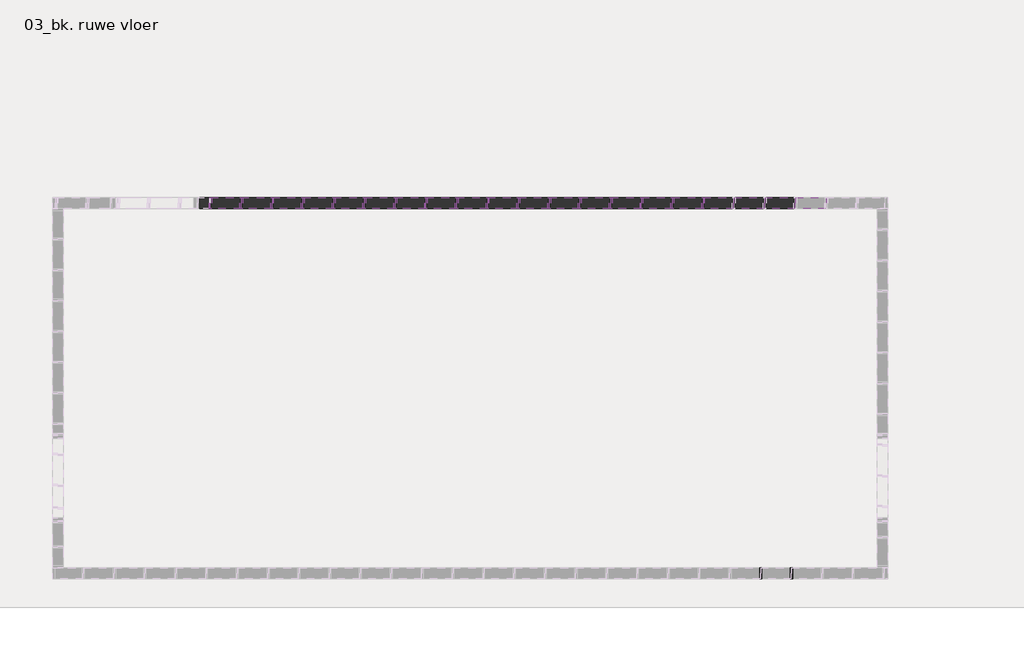
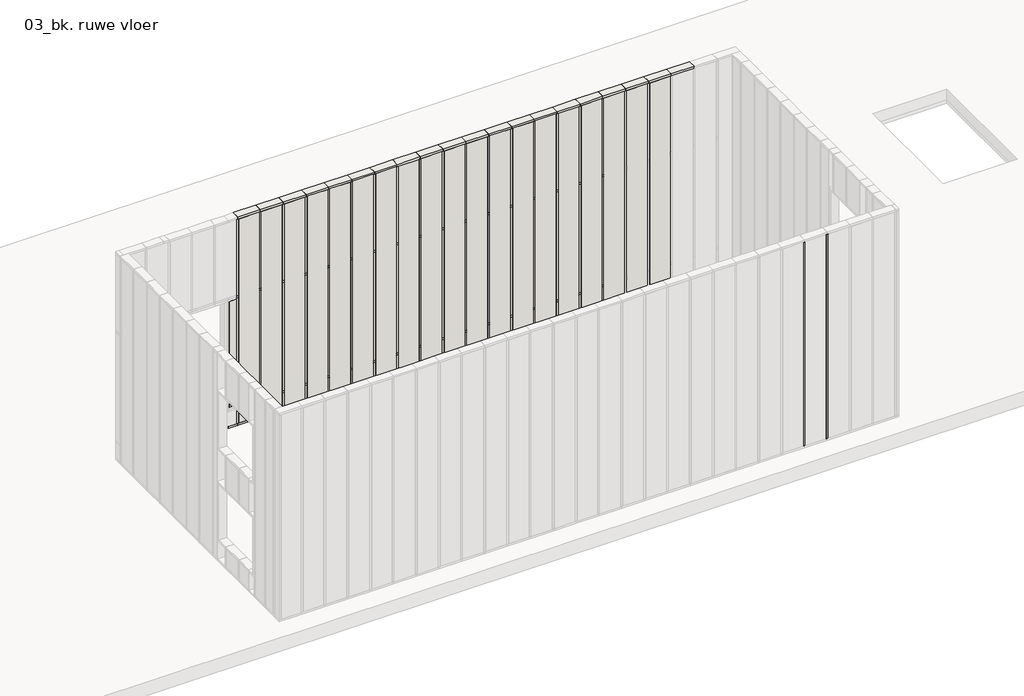
# One storey, part 3 of 9: 144 walls.
# Revit data of these elements (continued)
# Type "Rectangular Mullion : NLRS_21_CWM_hsb-regel 38x142_gen_rsf"
#   Type IfcGUID = "07M7mRoiH1CR8m_RSKIwpF"
#   Assembly Code = "21.10"
#   IfcExportAs = "IfcWall"
#   built-in parameter 1007322 = 0.465879 (stored number, unit not read)
#   built-in parameter 1007321 = 0.062336 (stored number, unit not read)
#   built-in parameter 1007320 = 0.062336 (stored number, unit not read)
# Type "System Panel : NLRS_21_CWP_hsb-vulling minerale wol 142 _gen_rsf"
#   Type IfcGUID = "07M7mRoiH1CR8m_RSKIwpC"
#   Assembly Code = "21.23"
#   IfcExportAs = "IfcWall"
# Element 1 (IfcWall, "Rectangular Mullion : NLRS_21_CWM_hsb-regel 38x142_gen_rsf")
#   IfcGUID = "07M7mRoiH1CR8m_RSKIwQK"
#   IsExternal = yes
#   LoadBearing = yes
#   Phase Created = NLRS_nieuw
#   Materials on its faces: "NLRS_i2_hout naaldhout vuren_gen_rsf"
# Element 2 (IfcWall, "Rectangular Mullion : NLRS_21_CWM_hsb-regel 38x142_gen_rsf")
#   IfcGUID = "07M7mRoiH1CR8m_RSKIwQR"
#   IsExternal = yes
#   LoadBearing = yes
#   Phase Created = NLRS_nieuw
#   Materials on its faces: "NLRS_i2_hout naaldhout vuren_gen_rsf"
# Element 3 (IfcWall, "Rectangular Mullion : NLRS_21_CWM_hsb-regel 38x142_gen_rsf")
#   IfcGUID = "07M7mRoiH1CR8m_RSKIwQQ"
#   IsExternal = yes
#   LoadBearing = yes
#   Phase Created = NLRS_nieuw
#   Materials on its faces: "NLRS_i2_hout naaldhout vuren_gen_rsf"
# Element 4 (IfcWall, "Rectangular Mullion : NLRS_21_CWM_hsb-regel 38x142_gen_rsf")
#   IfcGUID = "07M7mRoiH1CR8m_RSKIwQP"
#   IsExternal = yes
#   LoadBearing = yes
#   Phase Created = NLRS_nieuw
#   Materials on its faces: "NLRS_i2_hout naaldhout vuren_gen_rsf"
# Element 5 (IfcWall, "Rectangular Mullion : NLRS_21_CWM_hsb-regel 38x142_gen_rsf")
#   IfcGUID = "07M7mRoiH1CR8m_RSKIwQO"
#   IsExternal = yes
#   LoadBearing = yes
#   Phase Created = NLRS_nieuw
#   Materials on its faces: "NLRS_i2_hout naaldhout vuren_gen_rsf"
# Element 6 (IfcWall, "Rectangular Mullion : NLRS_21_CWM_hsb-regel 38x142_gen_rsf")
#   IfcGUID = "07M7mRoiH1CR8m_RSKIwQV"
#   IsExternal = yes
#   LoadBearing = yes
#   Phase Created = NLRS_nieuw
#   Materials on its faces: "NLRS_i2_hout naaldhout vuren_gen_rsf"
# Element 7 (IfcWall, "Rectangular Mullion : NLRS_21_CWM_hsb-regel 38x142_gen_rsf")
#   IfcGUID = "07M7mRoiH1CR8m_RSKIwQU"
#   IsExternal = yes
#   LoadBearing = yes
#   Phase Created = NLRS_nieuw
#   Materials on its faces: "NLRS_i2_hout naaldhout vuren_gen_rsf"
# Element 8 (IfcWall, "Rectangular Mullion : NLRS_21_CWM_hsb-regel 38x142_gen_rsf")
#   IfcGUID = "07M7mRoiH1CR8m_RSKIwQT"
#   IsExternal = yes
#   LoadBearing = yes
#   Phase Created = NLRS_nieuw
#   Materials on its faces: "NLRS_i2_hout naaldhout vuren_gen_rsf"
# Element 9 (IfcWall, "Rectangular Mullion : NLRS_21_CWM_hsb-regel 38x142_gen_rsf")
#   IfcGUID = "07M7mRoiH1CR8m_RSKIwQS"
#   IsExternal = yes
#   LoadBearing = yes
#   Phase Created = NLRS_nieuw
#   Materials on its faces: "NLRS_i2_hout naaldhout vuren_gen_rsf"
# Element 10 (IfcWall, "Rectangular Mullion : NLRS_21_CWM_hsb-regel 38x142_gen_rsf")
#   IfcGUID = "07M7mRoiH1CR8m_RSKIwPZ"
#   IsExternal = yes
#   LoadBearing = yes
#   Phase Created = NLRS_nieuw
#   Materials on its faces: "NLRS_i2_hout naaldhout vuren_gen_rsf"
# Element 11 (IfcWall, "Rectangular Mullion : NLRS_21_CWM_hsb-regel 38x142_gen_rsf")
#   IfcGUID = "07M7mRoiH1CR8m_RSKIwPY"
#   IsExternal = yes
#   LoadBearing = yes
#   Phase Created = NLRS_nieuw
#   Materials on its faces: "NLRS_i2_hout naaldhout vuren_gen_rsf"
# Element 12 (IfcWall, "Rectangular Mullion : NLRS_21_CWM_hsb-regel 38x142_gen_rsf")
#   IfcGUID = "07M7mRoiH1CR8m_RSKIwPX"
#   IsExternal = yes
#   LoadBearing = yes
#   Phase Created = NLRS_nieuw
#   Materials on its faces: "NLRS_i2_hout naaldhout vuren_gen_rsf"
# Element 13 (IfcWall, "Rectangular Mullion : NLRS_21_CWM_hsb-regel 38x142_gen_rsf")
#   IfcGUID = "07M7mRoiH1CR8m_RSKIwPW"
#   IsExternal = yes
#   LoadBearing = yes
#   Phase Created = NLRS_nieuw
#   Materials on its faces: "NLRS_i2_hout naaldhout vuren_gen_rsf"
# Element 14 (IfcWall, "Rectangular Mullion : NLRS_21_CWM_hsb-regel 38x142_gen_rsf")
#   IfcGUID = "07M7mRoiH1CR8m_RSKIwPd"
#   IsExternal = yes
#   LoadBearing = yes
#   Phase Created = NLRS_nieuw
#   Materials on its faces: "NLRS_i2_hout naaldhout vuren_gen_rsf"
# Element 15 (IfcWall, "Rectangular Mullion : NLRS_21_CWM_hsb-regel 38x142_gen_rsf")
#   IfcGUID = "07M7mRoiH1CR8m_RSKIwPc"
#   IsExternal = yes
#   LoadBearing = yes
#   Phase Created = NLRS_nieuw
#   Materials on its faces: "NLRS_i2_hout naaldhout vuren_gen_rsf"
# Element 16 (IfcWall, "Rectangular Mullion : NLRS_21_CWM_hsb-regel 38x142_gen_rsf")
#   IfcGUID = "07M7mRoiH1CR8m_RSKIwPb"
#   IsExternal = yes
#   LoadBearing = yes
#   Phase Created = NLRS_nieuw
#   Materials on its faces: "NLRS_i2_hout naaldhout vuren_gen_rsf"
# Element 17 (IfcWall, "Rectangular Mullion : NLRS_21_CWM_hsb-regel 38x142_gen_rsf")
#   IfcGUID = "07M7mRoiH1CR8m_RSKIwPa"
#   IsExternal = yes
#   LoadBearing = yes
#   Phase Created = NLRS_nieuw
#   Materials on its faces: "NLRS_i2_hout naaldhout vuren_gen_rsf"
# Element 18 (IfcWall, "Rectangular Mullion : NLRS_21_CWM_hsb-regel 38x142_gen_rsf")
#   IfcGUID = "07M7mRoiH1CR8m_RSKIwUD"
#   IsExternal = yes
#   LoadBearing = yes
#   Phase Created = NLRS_nieuw
#   Materials on its faces: "NLRS_i2_hout naaldhout vuren_gen_rsf"
# Element 19 (IfcWall, "Rectangular Mullion : NLRS_21_CWM_hsb-regel 38x142_gen_rsf")
#   IfcGUID = "07M7mRoiH1CR8m_RSKIwUC"
#   IsExternal = yes
#   LoadBearing = yes
#   Phase Created = NLRS_nieuw
#   Materials on its faces: "NLRS_i2_hout naaldhout vuren_gen_rsf"
# Element 20 (IfcWall, "Rectangular Mullion : NLRS_21_CWM_hsb-regel 38x142_gen_rsf")
#   IfcGUID = "07M7mRoiH1CR8m_RSKIwIM"
#   IsExternal = yes
#   LoadBearing = yes
#   Phase Created = NLRS_nieuw
#   Materials on its faces: "NLRS_i2_hout naaldhout vuren_gen_rsf"
# Element 21 (IfcWall, "Rectangular Mullion : NLRS_21_CWM_hsb-regel 38x142_gen_rsf")
#   IfcGUID = "07M7mRoiH1CR8m_RSKIwPj"
#   IsExternal = yes
#   LoadBearing = yes
#   Phase Created = NLRS_nieuw
#   Materials on its faces: "NLRS_i2_hout naaldhout vuren_gen_rsf"
# Element 22 (IfcWall, "Rectangular Mullion : NLRS_21_CWM_hsb-regel 38x142_gen_rsf")
#   IfcGUID = "07M7mRoiH1CR8m_RSKIwPi"
#   IsExternal = yes
#   LoadBearing = yes
#   Phase Created = NLRS_nieuw
#   Materials on its faces: "NLRS_i2_hout naaldhout vuren_gen_rsf"
# Element 23 (IfcWall, "Rectangular Mullion : NLRS_21_CWM_hsb-regel 38x142_gen_rsf")
#   IfcGUID = "07M7mRoiH1CR8m_RSKIwPp"
#   IsExternal = yes
#   LoadBearing = yes
#   Phase Created = NLRS_nieuw
#   Materials on its faces: "NLRS_i2_hout naaldhout vuren_gen_rsf"
# Element 24 (IfcWall, "Rectangular Mullion : NLRS_21_CWM_hsb-regel 38x142_gen_rsf")
#   IfcGUID = "07M7mRoiH1CR8m_RSKIwPo"
#   IsExternal = yes
#   LoadBearing = yes
#   Phase Created = NLRS_nieuw
#   Materials on its faces: "NLRS_i2_hout naaldhout vuren_gen_rsf"
# Element 25 (IfcWall, "Rectangular Mullion : NLRS_21_CWM_hsb-regel 38x142_gen_rsf")
#   IfcGUID = "07M7mRoiH1CR8m_RSKIwPn"
#   IsExternal = yes
#   LoadBearing = yes
#   Phase Created = NLRS_nieuw
#   Materials on its faces: "NLRS_i2_hout naaldhout vuren_gen_rsf"
# Element 26 (IfcWall, "Rectangular Mullion : NLRS_21_CWM_hsb-regel 38x142_gen_rsf")
#   IfcGUID = "07M7mRoiH1CR8m_RSKIwPm"
#   IsExternal = yes
#   LoadBearing = yes
#   Phase Created = NLRS_nieuw
#   Materials on its faces: "NLRS_i2_hout naaldhout vuren_gen_rsf"
# Element 27 (IfcWall, "Rectangular Mullion : NLRS_21_CWM_hsb-regel 38x142_gen_rsf")
#   IfcGUID = "07M7mRoiH1CR8m_RSKIwPt"
#   IsExternal = yes
#   LoadBearing = yes
#   Phase Created = NLRS_nieuw
#   Materials on its faces: "NLRS_i2_hout naaldhout vuren_gen_rsf"
# Element 28 (IfcWall, "Rectangular Mullion : NLRS_21_CWM_hsb-regel 38x142_gen_rsf")
#   IfcGUID = "07M7mRoiH1CR8m_RSKIwPs"
#   IsExternal = yes
#   LoadBearing = yes
#   Phase Created = NLRS_nieuw
#   Materials on its faces: "NLRS_i2_hout naaldhout vuren_gen_rsf"
# Element 29 (IfcWall, "Rectangular Mullion : NLRS_21_CWM_hsb-regel 38x142_gen_rsf")
#   IfcGUID = "07M7mRoiH1CR8m_RSKIwPr"
#   IsExternal = yes
#   LoadBearing = yes
#   Phase Created = NLRS_nieuw
#   Materials on its faces: "NLRS_i2_hout naaldhout vuren_gen_rsf"
# Element 30 (IfcWall, "Rectangular Mullion : NLRS_21_CWM_hsb-regel 38x142_gen_rsf")
#   IfcGUID = "07M7mRoiH1CR8m_RSKIwPq"
#   IsExternal = yes
#   LoadBearing = yes
#   Phase Created = NLRS_nieuw
#   Materials on its faces: "NLRS_i2_hout naaldhout vuren_gen_rsf"
# Element 31 (IfcWall, "Rectangular Mullion : NLRS_21_CWM_hsb-regel 38x142_gen_rsf")
#   IfcGUID = "07M7mRoiH1CR8m_RSKIwPx"
#   IsExternal = yes
#   LoadBearing = yes
#   Phase Created = NLRS_nieuw
#   Materials on its faces: "NLRS_i2_hout naaldhout vuren_gen_rsf"
# Element 32 (IfcWall, "Rectangular Mullion : NLRS_21_CWM_hsb-regel 38x142_gen_rsf")
#   IfcGUID = "07M7mRoiH1CR8m_RSKIwPw"
#   IsExternal = yes
#   LoadBearing = yes
#   Phase Created = NLRS_nieuw
#   Materials on its faces: "NLRS_i2_hout naaldhout vuren_gen_rsf"
# Element 33 (IfcWall, "Rectangular Mullion : NLRS_21_CWM_hsb-regel 38x142_gen_rsf")
#   IfcGUID = "07M7mRoiH1CR8m_RSKIwPv"
#   IsExternal = yes
#   LoadBearing = yes
#   Phase Created = NLRS_nieuw
#   Materials on its faces: "NLRS_i2_hout naaldhout vuren_gen_rsf"
# Element 34 (IfcWall, "Rectangular Mullion : NLRS_21_CWM_hsb-regel 38x142_gen_rsf")
#   IfcGUID = "07M7mRoiH1CR8m_RSKIwPu"
#   IsExternal = yes
#   LoadBearing = yes
#   Phase Created = NLRS_nieuw
#   Materials on its faces: "NLRS_i2_hout naaldhout vuren_gen_rsf"
# Element 35 (IfcWall, "Rectangular Mullion : NLRS_21_CWM_hsb-regel 38x142_gen_rsf")
#   IfcGUID = "07M7mRoiH1CR8m_RSKIwUJ"
#   IsExternal = yes
#   LoadBearing = yes
#   Phase Created = NLRS_nieuw
#   Materials on its faces: "NLRS_i2_hout naaldhout vuren_gen_rsf"
# Element 36 (IfcWall, "Rectangular Mullion : NLRS_21_CWM_hsb-regel 38x142_gen_rsf")
#   IfcGUID = "3JRv6RmLn4$9gi2tFo70EI"
#   IsExternal = yes
#   LoadBearing = yes
#   Phase Created = NLRS_nieuw
#   Materials on its faces: "NLRS_i2_hout naaldhout vuren_gen_rsf"
# Element 37 (IfcWall, "Rectangular Mullion : NLRS_21_CWM_hsb-regel 38x142_gen_rsf")
#   IfcGUID = "07M7mRoiH1CR8m_RSKIwIY"
#   IsExternal = yes
#   LoadBearing = yes
#   Phase Created = NLRS_nieuw
#   Materials on its faces: "NLRS_i2_hout naaldhout vuren_gen_rsf"
# Element 38 (IfcWall, "Rectangular Mullion : NLRS_21_CWM_hsb-regel 38x142_gen_rsf")
#   IfcGUID = "07M7mRoiH1CR8m_RSKIwIX"
#   IsExternal = yes
#   LoadBearing = yes
#   Phase Created = NLRS_nieuw
#   Materials on its faces: "NLRS_i2_hout naaldhout vuren_gen_rsf"
# Element 39 (IfcWall, "Rectangular Mullion : NLRS_21_CWM_hsb-regel 38x142_gen_rsf")
#   IfcGUID = "07M7mRoiH1CR8m_RSKIwP0"
#   IsExternal = yes
#   LoadBearing = yes
#   Phase Created = NLRS_nieuw
#   Materials on its faces: "NLRS_i2_hout naaldhout vuren_gen_rsf"
# Element 40 (IfcWall, "Rectangular Mullion : NLRS_21_CWM_hsb-regel 38x142_gen_rsf")
#   IfcGUID = "07M7mRoiH1CR8m_RSKIwP7"
#   IsExternal = yes
#   LoadBearing = yes
#   Phase Created = NLRS_nieuw
#   Materials on its faces: "NLRS_i2_hout naaldhout vuren_gen_rsf"
# Element 41 (IfcWall, "Rectangular Mullion : NLRS_21_CWM_hsb-regel 38x142_gen_rsf")
#   IfcGUID = "07M7mRoiH1CR8m_RSKIwP6"
#   IsExternal = yes
#   LoadBearing = yes
#   Phase Created = NLRS_nieuw
#   Materials on its faces: "NLRS_i2_hout naaldhout vuren_gen_rsf"
# Element 42 (IfcWall, "Rectangular Mullion : NLRS_21_CWM_hsb-regel 38x142_gen_rsf")
#   IfcGUID = "07M7mRoiH1CR8m_RSKIwP5"
#   IsExternal = yes
#   LoadBearing = yes
#   Phase Created = NLRS_nieuw
#   Materials on its faces: "NLRS_i2_hout naaldhout vuren_gen_rsf"
# Element 43 (IfcWall, "Rectangular Mullion : NLRS_21_CWM_hsb-regel 38x142_gen_rsf")
#   IfcGUID = "07M7mRoiH1CR8m_RSKIwP4"
#   IsExternal = yes
#   LoadBearing = yes
#   Phase Created = NLRS_nieuw
#   Materials on its faces: "NLRS_i2_hout naaldhout vuren_gen_rsf"
# Element 44 (IfcWall, "Rectangular Mullion : NLRS_21_CWM_hsb-regel 38x142_gen_rsf")
#   IfcGUID = "07M7mRoiH1CR8m_RSKIwPB"
#   IsExternal = yes
#   LoadBearing = yes
#   Phase Created = NLRS_nieuw
#   Materials on its faces: "NLRS_i2_hout naaldhout vuren_gen_rsf"
# Element 45 (IfcWall, "Rectangular Mullion : NLRS_21_CWM_hsb-regel 38x142_gen_rsf")
#   IfcGUID = "07M7mRoiH1CR8m_RSKIwPA"
#   IsExternal = yes
#   LoadBearing = yes
#   Phase Created = NLRS_nieuw
#   Materials on its faces: "NLRS_i2_hout naaldhout vuren_gen_rsf"
# Element 46 (IfcWall, "Rectangular Mullion : NLRS_21_CWM_hsb-regel 38x142_gen_rsf")
#   IfcGUID = "07M7mRoiH1CR8m_RSKIwP9"
#   IsExternal = yes
#   LoadBearing = yes
#   Phase Created = NLRS_nieuw
#   Materials on its faces: "NLRS_i2_hout naaldhout vuren_gen_rsf"
# Element 47 (IfcWall, "Rectangular Mullion : NLRS_21_CWM_hsb-regel 38x142_gen_rsf")
#   IfcGUID = "07M7mRoiH1CR8m_RSKIwP8"
#   IsExternal = yes
#   LoadBearing = yes
#   Phase Created = NLRS_nieuw
#   Materials on its faces: "NLRS_i2_hout naaldhout vuren_gen_rsf"
# Element 48 (IfcWall, "Rectangular Mullion : NLRS_21_CWM_hsb-regel 38x142_gen_rsf")
#   IfcGUID = "07M7mRoiH1CR8m_RSKIwPF"
#   IsExternal = yes
#   LoadBearing = yes
#   Phase Created = NLRS_nieuw
#   Materials on its faces: "NLRS_i2_hout naaldhout vuren_gen_rsf"
# Element 49 (IfcWall, "Rectangular Mullion : NLRS_21_CWM_hsb-regel 38x142_gen_rsf")
#   IfcGUID = "07M7mRoiH1CR8m_RSKIwPE"
#   IsExternal = yes
#   LoadBearing = yes
#   Phase Created = NLRS_nieuw
#   Materials on its faces: "NLRS_i2_hout naaldhout vuren_gen_rsf"
# Element 50 (IfcWall, "Rectangular Mullion : NLRS_21_CWM_hsb-regel 38x142_gen_rsf")
#   IfcGUID = "07M7mRoiH1CR8m_RSKIwPD"
#   IsExternal = yes
#   LoadBearing = yes
#   Phase Created = NLRS_nieuw
#   Materials on its faces: "NLRS_i2_hout naaldhout vuren_gen_rsf"
# Element 51 (IfcWall, "Rectangular Mullion : NLRS_21_CWM_hsb-regel 38x142_gen_rsf")
#   IfcGUID = "07M7mRoiH1CR8m_RSKIwPC"
#   IsExternal = yes
#   LoadBearing = yes
#   Phase Created = NLRS_nieuw
#   Materials on its faces: "NLRS_i2_hout naaldhout vuren_gen_rsf"
# Element 52 (IfcWall, "Rectangular Mullion : NLRS_21_CWM_hsb-regel 38x142_gen_rsf")
#   IfcGUID = "07M7mRoiH1CR8m_RSKIwPJ"
#   IsExternal = yes
#   LoadBearing = yes
#   Phase Created = NLRS_nieuw
#   Materials on its faces: "NLRS_i2_hout naaldhout vuren_gen_rsf"
# Element 53 (IfcWall, "Rectangular Mullion : NLRS_21_CWM_hsb-regel 38x142_gen_rsf")
#   IfcGUID = "07M7mRoiH1CR8m_RSKIwUI"
#   IsExternal = yes
#   LoadBearing = yes
#   Phase Created = NLRS_nieuw
#   Materials on its faces: "NLRS_i2_hout naaldhout vuren_gen_rsf"
# Element 54 (IfcWall, "Rectangular Mullion : NLRS_21_CWM_hsb-regel 38x142_gen_rsf")
#   IfcGUID = "07M7mRoiH1CR8m_RSKIwUH"
#   IsExternal = yes
#   LoadBearing = yes
#   Phase Created = NLRS_nieuw
#   Materials on its faces: "NLRS_i2_hout naaldhout vuren_gen_rsf"
# Element 55 (IfcWall, "Rectangular Mullion : NLRS_21_CWM_hsb-regel 38x142_gen_rsf")
#   IfcGUID = "07M7mRoiH1CR8m_RSKIwHY"
#   IsExternal = yes
#   LoadBearing = yes
#   Phase Created = NLRS_nieuw
#   Materials on its faces: "NLRS_i2_hout naaldhout vuren_gen_rsf"
# Element 56 (IfcWall, "Rectangular Mullion : NLRS_21_CWM_hsb-regel 38x142_gen_rsf")
#   IfcGUID = "3JRv6RmLn4$9gi2tFo70EJ"
#   IsExternal = yes
#   LoadBearing = yes
#   Phase Created = NLRS_nieuw
#   Materials on its faces: "NLRS_i2_hout naaldhout vuren_gen_rsf"
# Element 57 (IfcWall, "Rectangular Mullion : NLRS_21_CWM_hsb-regel 38x142_gen_rsf")
#   IfcGUID = "3JRv6RmLn4$9gi2tFo70WL"
#   IsExternal = yes
#   LoadBearing = yes
#   Phase Created = NLRS_nieuw
#   Materials on its faces: "NLRS_i2_hout naaldhout vuren_gen_rsf"
# Element 58 (IfcWall, "Rectangular Mullion : NLRS_21_CWM_hsb-regel 38x142_gen_rsf")
#   IfcGUID = "3JRv6RmLn4$9gi2tFo70WM"
#   IsExternal = yes
#   LoadBearing = yes
#   Phase Created = NLRS_nieuw
#   Materials on its faces: "NLRS_i2_hout naaldhout vuren_gen_rsf"
# Element 59 (IfcWall, "Rectangular Mullion : NLRS_21_CWM_hsb-regel 38x142_gen_rsf")
#   IfcGUID = "3JRv6RmLn4$9gi2tFo70WN"
#   IsExternal = yes
#   LoadBearing = yes
#   Phase Created = NLRS_nieuw
#   Materials on its faces: "NLRS_i2_hout naaldhout vuren_gen_rsf"
# Element 60 (IfcWall, "Rectangular Mullion : NLRS_21_CWM_hsb-regel 38x142_gen_rsf")
#   IfcGUID = "3JRv6RmLn4$9gi2tFo70WG"
#   IsExternal = yes
#   LoadBearing = yes
#   Phase Created = NLRS_nieuw
#   Materials on its faces: "NLRS_i2_hout naaldhout vuren_gen_rsf"
# Element 61 (IfcWall, "Rectangular Mullion : NLRS_21_CWM_hsb-regel 38x142_gen_rsf")
#   IfcGUID = "3JRv6RmLn4$9gi2tFo70WH"
#   IsExternal = yes
#   LoadBearing = yes
#   Phase Created = NLRS_nieuw
#   Materials on its faces: "NLRS_i2_hout naaldhout vuren_gen_rsf"
# Element 62 (IfcWall, "Rectangular Mullion : NLRS_21_CWM_hsb-regel 38x142_gen_rsf")
#   IfcGUID = "3JRv6RmLn4$9gi2tFo70WI"
#   IsExternal = yes
#   LoadBearing = yes
#   Phase Created = NLRS_nieuw
#   Materials on its faces: "NLRS_i2_hout naaldhout vuren_gen_rsf"
# Element 63 (IfcWall, "Rectangular Mullion : NLRS_21_CWM_hsb-regel 38x142_gen_rsf")
#   IfcGUID = "3JRv6RmLn4$9gi2tFo70WJ"
#   IsExternal = yes
#   LoadBearing = yes
#   Phase Created = NLRS_nieuw
#   Materials on its faces: "NLRS_i2_hout naaldhout vuren_gen_rsf"
# Element 64 (IfcWall, "Rectangular Mullion : NLRS_21_CWM_hsb-regel 38x142_gen_rsf")
#   IfcGUID = "3JRv6RmLn4$9gi2tFo70WS"
#   IsExternal = yes
#   LoadBearing = yes
#   Phase Created = NLRS_nieuw
#   Materials on its faces: "NLRS_i2_hout naaldhout vuren_gen_rsf"
# Element 65 (IfcWall, "Rectangular Mullion : NLRS_21_CWM_hsb-regel 38x142_gen_rsf")
#   IfcGUID = "3JRv6RmLn4$9gi2tFo70WT"
#   IsExternal = yes
#   LoadBearing = yes
#   Phase Created = NLRS_nieuw
#   Materials on its faces: "NLRS_i2_hout naaldhout vuren_gen_rsf"
# Element 66 (IfcWall, "Rectangular Mullion : NLRS_21_CWM_hsb-regel 38x142_gen_rsf")
#   IfcGUID = "3JRv6RmLn4$9gi2tFo70WU"
#   IsExternal = yes
#   LoadBearing = yes
#   Phase Created = NLRS_nieuw
#   Materials on its faces: "NLRS_i2_hout naaldhout vuren_gen_rsf"
# Element 67 (IfcWall, "Rectangular Mullion : NLRS_21_CWM_hsb-regel 38x142_gen_rsf")
#   IfcGUID = "3JRv6RmLn4$9gi2tFo70WV"
#   IsExternal = yes
#   LoadBearing = yes
#   Phase Created = NLRS_nieuw
#   Materials on its faces: "NLRS_i2_hout naaldhout vuren_gen_rsf"
# Element 68 (IfcWall, "Rectangular Mullion : NLRS_21_CWM_hsb-regel 38x142_gen_rsf")
#   IfcGUID = "3JRv6RmLn4$9gi2tFo70WO"
#   IsExternal = yes
#   LoadBearing = yes
#   Phase Created = NLRS_nieuw
#   Materials on its faces: "NLRS_i2_hout naaldhout vuren_gen_rsf"
# Element 69 (IfcWall, "Rectangular Mullion : NLRS_21_CWM_hsb-regel 38x142_gen_rsf")
#   IfcGUID = "3JRv6RmLn4$9gi2tFo70WP"
#   IsExternal = yes
#   LoadBearing = yes
#   Phase Created = NLRS_nieuw
#   Materials on its faces: "NLRS_i2_hout naaldhout vuren_gen_rsf"
# Element 70 (IfcWall, "Rectangular Mullion : NLRS_21_CWM_hsb-regel 38x142_gen_rsf")
#   IfcGUID = "3JRv6RmLn4$9gi2tFo70WQ"
#   IsExternal = yes
#   LoadBearing = yes
#   Phase Created = NLRS_nieuw
#   Materials on its faces: "NLRS_i2_hout naaldhout vuren_gen_rsf"
# Element 71 (IfcWall, "Rectangular Mullion : NLRS_21_CWM_hsb-regel 38x142_gen_rsf")
#   IfcGUID = "3JRv6RmLn4$9gi2tFo70WR"
#   IsExternal = yes
#   LoadBearing = yes
#   Phase Created = NLRS_nieuw
#   Materials on its faces: "NLRS_i2_hout naaldhout vuren_gen_rsf"
# Element 72 (IfcWall, "Rectangular Mullion : NLRS_21_CWM_hsb-regel 38x142_gen_rsf")
#   IfcGUID = "3JRv6RmLn4$9gi2tFo70Xa"
#   IsExternal = yes
#   LoadBearing = yes
#   Phase Created = NLRS_nieuw
#   Materials on its faces: "NLRS_i2_hout naaldhout vuren_gen_rsf"
# Element 73 (IfcWall, "Rectangular Mullion : NLRS_21_CWM_hsb-regel 38x142_gen_rsf")
#   IfcGUID = "3JRv6RmLn4$9gi2tFo70Xb"
#   IsExternal = yes
#   LoadBearing = yes
#   Phase Created = NLRS_nieuw
#   Materials on its faces: "NLRS_i2_hout naaldhout vuren_gen_rsf"
# Element 74 (IfcWall, "Rectangular Mullion : NLRS_21_CWM_hsb-regel 38x142_gen_rsf")
#   IfcGUID = "3JRv6RmLn4$9gi2tFo70wj"
#   IsExternal = yes
#   LoadBearing = yes
#   Phase Created = NLRS_nieuw
#   Materials on its faces: "NLRS_i2_hout naaldhout vuren_gen_rsf"
# Element 75 (IfcWall, "Rectangular Mullion : NLRS_21_CWM_hsb-regel 38x142_gen_rsf")
#   IfcGUID = "3JRv6RmLn4$9gi2tFo70wk"
#   IsExternal = yes
#   LoadBearing = yes
#   Phase Created = NLRS_nieuw
#   Materials on its faces: "NLRS_i2_hout naaldhout vuren_gen_rsf"
# Element 76 (IfcWall, "Rectangular Mullion : NLRS_21_CWM_hsb-regel 38x142_gen_rsf")
#   IfcGUID = "3JRv6RmLn4$9gi2tFo70wl"
#   IsExternal = yes
#   LoadBearing = yes
#   Phase Created = NLRS_nieuw
#   Materials on its faces: "NLRS_i2_hout naaldhout vuren_gen_rsf"
# Element 77 (IfcWall, "Rectangular Mullion : NLRS_21_CWM_hsb-regel 38x142_gen_rsf")
#   IfcGUID = "3JRv6RmLn4$9gi2tFo70we"
#   IsExternal = yes
#   LoadBearing = yes
#   Phase Created = NLRS_nieuw
#   Materials on its faces: "NLRS_i2_hout naaldhout vuren_gen_rsf"
# Element 78 (IfcWall, "Rectangular Mullion : NLRS_21_CWM_hsb-regel 38x142_gen_rsf")
#   IfcGUID = "3JRv6RmLn4$9gi2tFo70wf"
#   IsExternal = yes
#   LoadBearing = yes
#   Phase Created = NLRS_nieuw
#   Materials on its faces: "NLRS_i2_hout naaldhout vuren_gen_rsf"
# Element 79 (IfcWall, "Rectangular Mullion : NLRS_21_CWM_hsb-regel 38x142_gen_rsf")
#   IfcGUID = "3JRv6RmLn4$9gi2tFo70wg"
#   IsExternal = yes
#   LoadBearing = yes
#   Phase Created = NLRS_nieuw
#   Materials on its faces: "NLRS_i2_hout naaldhout vuren_gen_rsf"
# Element 80 (IfcWall, "Rectangular Mullion : NLRS_21_CWM_hsb-regel 38x142_gen_rsf")
#   IfcGUID = "3JRv6RmLn4$9gi2tFo70wh"
#   IsExternal = yes
#   LoadBearing = yes
#   Phase Created = NLRS_nieuw
#   Materials on its faces: "NLRS_i2_hout naaldhout vuren_gen_rsf"
# Element 81 (IfcWall, "Rectangular Mullion : NLRS_21_CWM_hsb-regel 38x142_gen_rsf")
#   IfcGUID = "3JRv6RmLn4$9gi2tFo70wq"
#   IsExternal = yes
#   LoadBearing = yes
#   Phase Created = NLRS_nieuw
#   Materials on its faces: "NLRS_i2_hout naaldhout vuren_gen_rsf"
# Element 82 (IfcWall, "Rectangular Mullion : NLRS_21_CWM_hsb-regel 38x142_gen_rsf")
#   IfcGUID = "3JRv6RmLn4$9gi2tFo70wr"
#   IsExternal = yes
#   LoadBearing = yes
#   Phase Created = NLRS_nieuw
#   Materials on its faces: "NLRS_i2_hout naaldhout vuren_gen_rsf"
# Element 83 (IfcWall, "Rectangular Mullion : NLRS_21_CWM_hsb-regel 38x142_gen_rsf")
#   IfcGUID = "3JRv6RmLn4$9gi2tFo70ws"
#   IsExternal = yes
#   LoadBearing = yes
#   Phase Created = NLRS_nieuw
#   Materials on its faces: "NLRS_i2_hout naaldhout vuren_gen_rsf"
# Element 84 (IfcWall, "Rectangular Mullion : NLRS_21_CWM_hsb-regel 38x142_gen_rsf")
#   IfcGUID = "3JRv6RmLn4$9gi2tFo70wt"
#   IsExternal = yes
#   LoadBearing = yes
#   Phase Created = NLRS_nieuw
#   Materials on its faces: "NLRS_i2_hout naaldhout vuren_gen_rsf"
# Element 85 (IfcWall, "Rectangular Mullion : NLRS_21_CWM_hsb-regel 38x142_gen_rsf")
#   IfcGUID = "3JRv6RmLn4$9gi2tFo70wm"
#   IsExternal = yes
#   LoadBearing = yes
#   Phase Created = NLRS_nieuw
#   Materials on its faces: "NLRS_i2_hout naaldhout vuren_gen_rsf"
# Element 86 (IfcWall, "Rectangular Mullion : NLRS_21_CWM_hsb-regel 38x142_gen_rsf")
#   IfcGUID = "3JRv6RmLn4$9gi2tFo70wn"
#   IsExternal = yes
#   LoadBearing = yes
#   Phase Created = NLRS_nieuw
#   Materials on its faces: "NLRS_i2_hout naaldhout vuren_gen_rsf"
# Element 87 (IfcWall, "Rectangular Mullion : NLRS_21_CWM_hsb-regel 38x142_gen_rsf")
#   IfcGUID = "3JRv6RmLn4$9gi2tFo70wo"
#   IsExternal = yes
#   LoadBearing = yes
#   Phase Created = NLRS_nieuw
#   Materials on its faces: "NLRS_i2_hout naaldhout vuren_gen_rsf"
# Element 88 (IfcWall, "Rectangular Mullion : NLRS_21_CWM_hsb-regel 38x142_gen_rsf")
#   IfcGUID = "3JRv6RmLn4$9gi2tFo70wp"
#   IsExternal = yes
#   LoadBearing = yes
#   Phase Created = NLRS_nieuw
#   Materials on its faces: "NLRS_i2_hout naaldhout vuren_gen_rsf"
# Element 89 (IfcWall, "Rectangular Mullion : NLRS_21_CWM_hsb-regel 38x142_gen_rsf")
#   IfcGUID = "3JRv6RmLn4$9gi2tFo70wy"
#   IsExternal = yes
#   LoadBearing = yes
#   Phase Created = NLRS_nieuw
#   Materials on its faces: "NLRS_i2_hout naaldhout vuren_gen_rsf"
# Element 90 (IfcWall, "Rectangular Mullion : NLRS_21_CWM_hsb-regel 38x142_gen_rsf")
#   IfcGUID = "3JRv6RmLn4$9gi2tFo70hi"
#   IsExternal = yes
#   LoadBearing = yes
#   Phase Created = NLRS_nieuw
#   Materials on its faces: "NLRS_i2_hout naaldhout vuren_gen_rsf"
# Element 91 (IfcWall, "Rectangular Mullion : NLRS_21_CWM_hsb-regel 38x142_gen_rsf")
#   IfcGUID = "3JRv6RmLn4$9gi2tFo70hj"
#   IsExternal = yes
#   LoadBearing = yes
#   Phase Created = NLRS_nieuw
#   Materials on its faces: "NLRS_i2_hout naaldhout vuren_gen_rsf"
# Element 92 (IfcWall, "Rectangular Mullion : NLRS_21_CWM_hsb-regel 38x142_gen_rsf")
#   IfcGUID = "3JRv6RmLn4$9gi2tFo70hk"
#   IsExternal = yes
#   LoadBearing = yes
#   Phase Created = NLRS_nieuw
#   Materials on its faces: "NLRS_i2_hout naaldhout vuren_gen_rsf"
# Element 93 (IfcWall, "Rectangular Mullion : NLRS_21_CWM_hsb-regel 38x142_gen_rsf")
#   IfcGUID = "3JRv6RmLn4$9gi2tFo70hl"
#   IsExternal = yes
#   LoadBearing = yes
#   Phase Created = NLRS_nieuw
#   Materials on its faces: "NLRS_i2_hout naaldhout vuren_gen_rsf"
# Element 94 (IfcWall, "Rectangular Mullion : NLRS_21_CWM_hsb-regel 38x142_gen_rsf")
#   IfcGUID = "3JRv6RmLn4$9gi2tFo70he"
#   IsExternal = yes
#   LoadBearing = yes
#   Phase Created = NLRS_nieuw
#   Materials on its faces: "NLRS_i2_hout naaldhout vuren_gen_rsf"
# Element 95 (IfcWall, "Rectangular Mullion : NLRS_21_CWM_hsb-regel 38x142_gen_rsf")
#   IfcGUID = "3JRv6RmLn4$9gi2tFo70hf"
#   IsExternal = yes
#   LoadBearing = yes
#   Phase Created = NLRS_nieuw
#   Materials on its faces: "NLRS_i2_hout naaldhout vuren_gen_rsf"
# Element 96 (IfcWall, "Rectangular Mullion : NLRS_21_CWM_hsb-regel 38x142_gen_rsf")
#   IfcGUID = "3JRv6RmLn4$9gi2tFo70hg"
#   IsExternal = yes
#   LoadBearing = yes
#   Phase Created = NLRS_nieuw
#   Materials on its faces: "NLRS_i2_hout naaldhout vuren_gen_rsf"
# Element 97 (IfcWall, "Rectangular Mullion : NLRS_21_CWM_hsb-regel 38x142_gen_rsf")
#   IfcGUID = "3JRv6RmLn4$9gi2tFo70hh"
#   IsExternal = yes
#   LoadBearing = yes
#   Phase Created = NLRS_nieuw
#   Materials on its faces: "NLRS_i2_hout naaldhout vuren_gen_rsf"
# Element 98 (IfcWall, "Rectangular Mullion : NLRS_21_CWM_hsb-regel 38x142_gen_rsf")
#   IfcGUID = "3JRv6RmLn4$9gi2tFo70hq"
#   IsExternal = yes
#   LoadBearing = yes
#   Phase Created = NLRS_nieuw
#   Materials on its faces: "NLRS_i2_hout naaldhout vuren_gen_rsf"
# Element 99 (IfcWall, "Rectangular Mullion : NLRS_21_CWM_hsb-regel 38x142_gen_rsf")
#   IfcGUID = "3JRv6RmLn4$9gi2tFo70hr"
#   IsExternal = yes
#   LoadBearing = yes
#   Phase Created = NLRS_nieuw
#   Materials on its faces: "NLRS_i2_hout naaldhout vuren_gen_rsf"
# Element 100 (IfcWall, "Rectangular Mullion : NLRS_21_CWM_hsb-regel 38x142_gen_rsf")
#   IfcGUID = "3JRv6RmLn4$9gi2tFo70hs"
#   IsExternal = yes
#   LoadBearing = yes
#   Phase Created = NLRS_nieuw
#   Materials on its faces: "NLRS_i2_hout naaldhout vuren_gen_rsf"
# Element 101 (IfcWall, "Rectangular Mullion : NLRS_21_CWM_hsb-regel 38x142_gen_rsf")
#   IfcGUID = "3JRv6RmLn4$9gi2tFo70ht"
#   IsExternal = yes
#   LoadBearing = yes
#   Phase Created = NLRS_nieuw
#   Materials on its faces: "NLRS_i2_hout naaldhout vuren_gen_rsf"
# Element 102 (IfcWall, "Rectangular Mullion : NLRS_21_CWM_hsb-regel 38x142_gen_rsf")
#   IfcGUID = "3JRv6RmLn4$9gi2tFo70hm"
#   IsExternal = yes
#   LoadBearing = yes
#   Phase Created = NLRS_nieuw
#   Materials on its faces: "NLRS_i2_hout naaldhout vuren_gen_rsf"
# Element 103 (IfcWall, "Rectangular Mullion : NLRS_21_CWM_hsb-regel 38x142_gen_rsf")
#   IfcGUID = "3JRv6RmLn4$9gi2tFo70hn"
#   IsExternal = yes
#   LoadBearing = yes
#   Phase Created = NLRS_nieuw
#   Materials on its faces: "NLRS_i2_hout naaldhout vuren_gen_rsf"
# Element 104 (IfcWall, "Rectangular Mullion : NLRS_21_CWM_hsb-regel 38x142_gen_rsf")
#   IfcGUID = "3JRv6RmLn4$9gi2tFo70ho"
#   IsExternal = yes
#   LoadBearing = yes
#   Phase Created = NLRS_nieuw
#   Materials on its faces: "NLRS_i2_hout naaldhout vuren_gen_rsf"
# Element 105 (IfcWall, "Rectangular Mullion : NLRS_21_CWM_hsb-regel 38x142_gen_rsf")
#   IfcGUID = "3JRv6RmLn4$9gi2tFo70hp"
#   IsExternal = yes
#   LoadBearing = yes
#   Phase Created = NLRS_nieuw
#   Materials on its faces: "NLRS_i2_hout naaldhout vuren_gen_rsf"
# Element 106 (IfcWall, "Rectangular Mullion : NLRS_21_CWM_hsb-regel 38x142_gen_rsf")
#   IfcGUID = "3JRv6RmLn4$9gi2tFo70wz"
#   IsExternal = yes
#   LoadBearing = yes
#   Phase Created = NLRS_nieuw
#   Materials on its faces: "NLRS_i2_hout naaldhout vuren_gen_rsf"
# Element 107 (IfcWall, "Rectangular Mullion : NLRS_21_CWM_hsb-regel 38x142_gen_rsf")
#   IfcGUID = "3JRv6RmLn4$9gi2tFo70hy"
#   IsExternal = yes
#   LoadBearing = yes
#   Phase Created = NLRS_nieuw
#   Materials on its faces: "NLRS_i2_hout naaldhout vuren_gen_rsf"
# Element 108 (IfcWall, "Rectangular Mullion : NLRS_21_CWM_hsb-regel 38x142_gen_rsf")
#   IfcGUID = "3JRv6RmLn4$9gi2tFo70kv"
#   IsExternal = yes
#   LoadBearing = yes
#   Phase Created = NLRS_nieuw
#   Materials on its faces: "NLRS_i2_hout naaldhout vuren_gen_rsf"
# Element 109 (IfcWall, "Rectangular Mullion : NLRS_21_CWM_hsb-regel 38x142_gen_rsf")
#   IfcGUID = "3JRv6RmLn4$9gi2tFo70kw"
#   IsExternal = yes
#   LoadBearing = yes
#   Phase Created = NLRS_nieuw
#   Materials on its faces: "NLRS_i2_hout naaldhout vuren_gen_rsf"
# Element 110 (IfcWall, "Rectangular Mullion : NLRS_21_CWM_hsb-regel 38x142_gen_rsf")
#   IfcGUID = "3JRv6RmLn4$9gi2tFo70kx"
#   IsExternal = yes
#   LoadBearing = yes
#   Phase Created = NLRS_nieuw
#   Materials on its faces: "NLRS_i2_hout naaldhout vuren_gen_rsf"
# Element 111 (IfcWall, "Rectangular Mullion : NLRS_21_CWM_hsb-regel 38x142_gen_rsf")
#   IfcGUID = "3JRv6RmLn4$9gi2tFo70k4"
#   IsExternal = yes
#   LoadBearing = yes
#   Phase Created = NLRS_nieuw
#   Materials on its faces: "NLRS_i2_hout naaldhout vuren_gen_rsf"
# Element 112 (IfcWall, "Rectangular Mullion : NLRS_21_CWM_hsb-regel 38x142_gen_rsf")
#   IfcGUID = "3JRv6RmLn4$9gi2tFo70k5"
#   IsExternal = yes
#   LoadBearing = yes
#   Phase Created = NLRS_nieuw
#   Materials on its faces: "NLRS_i2_hout naaldhout vuren_gen_rsf"
# Element 113 (IfcWall, "Rectangular Mullion : NLRS_21_CWM_hsb-regel 38x142_gen_rsf")
#   IfcGUID = "3JRv6RmLn4$9gi2tFo70k6"
#   IsExternal = yes
#   LoadBearing = yes
#   Phase Created = NLRS_nieuw
#   Materials on its faces: "NLRS_i2_hout naaldhout vuren_gen_rsf"
# Element 114 (IfcWall, "Rectangular Mullion : NLRS_21_CWM_hsb-regel 38x142_gen_rsf")
#   IfcGUID = "3JRv6RmLn4$9gi2tFo70k7"
#   IsExternal = yes
#   LoadBearing = yes
#   Phase Created = NLRS_nieuw
#   Materials on its faces: "NLRS_i2_hout naaldhout vuren_gen_rsf"
# Element 115 (IfcWall, "Rectangular Mullion : NLRS_21_CWM_hsb-regel 38x142_gen_rsf")
#   IfcGUID = "3JRv6RmLn4$9gi2tFo70k0"
#   IsExternal = yes
#   LoadBearing = yes
#   Phase Created = NLRS_nieuw
#   Materials on its faces: "NLRS_i2_hout naaldhout vuren_gen_rsf"
# Element 116 (IfcWall, "Rectangular Mullion : NLRS_21_CWM_hsb-regel 38x142_gen_rsf")
#   IfcGUID = "3JRv6RmLn4$9gi2tFo70k1"
#   IsExternal = yes
#   LoadBearing = yes
#   Phase Created = NLRS_nieuw
#   Materials on its faces: "NLRS_i2_hout naaldhout vuren_gen_rsf"
# Element 117 (IfcWall, "Rectangular Mullion : NLRS_21_CWM_hsb-regel 38x142_gen_rsf")
#   IfcGUID = "3JRv6RmLn4$9gi2tFo70k2"
#   IsExternal = yes
#   LoadBearing = yes
#   Phase Created = NLRS_nieuw
#   Materials on its faces: "NLRS_i2_hout naaldhout vuren_gen_rsf"
# Element 118 (IfcWall, "Rectangular Mullion : NLRS_21_CWM_hsb-regel 38x142_gen_rsf")
#   IfcGUID = "3JRv6RmLn4$9gi2tFo70k3"
#   IsExternal = yes
#   LoadBearing = yes
#   Phase Created = NLRS_nieuw
#   Materials on its faces: "NLRS_i2_hout naaldhout vuren_gen_rsf"
# Element 119 (IfcWall, "Rectangular Mullion : NLRS_21_CWM_hsb-regel 38x142_gen_rsf")
#   IfcGUID = "3JRv6RmLn4$9gi2tFo70kC"
#   IsExternal = yes
#   LoadBearing = yes
#   Phase Created = NLRS_nieuw
#   Materials on its faces: "NLRS_i2_hout naaldhout vuren_gen_rsf"
# Element 120 (IfcWall, "Rectangular Mullion : NLRS_21_CWM_hsb-regel 38x142_gen_rsf")
#   IfcGUID = "3JRv6RmLn4$9gi2tFo70kD"
#   IsExternal = yes
#   LoadBearing = yes
#   Phase Created = NLRS_nieuw
#   Materials on its faces: "NLRS_i2_hout naaldhout vuren_gen_rsf"
# Element 121 (IfcWall, "Rectangular Mullion : NLRS_21_CWM_hsb-regel 38x142_gen_rsf")
#   IfcGUID = "3JRv6RmLn4$9gi2tFo70kE"
#   IsExternal = yes
#   LoadBearing = yes
#   Phase Created = NLRS_nieuw
#   Materials on its faces: "NLRS_i2_hout naaldhout vuren_gen_rsf"
# Element 122 (IfcWall, "Rectangular Mullion : NLRS_21_CWM_hsb-regel 38x142_gen_rsf")
#   IfcGUID = "3JRv6RmLn4$9gi2tFo70kF"
#   IsExternal = yes
#   LoadBearing = yes
#   Phase Created = NLRS_nieuw
#   Materials on its faces: "NLRS_i2_hout naaldhout vuren_gen_rsf"
# Element 123 (IfcWall, "Rectangular Mullion : NLRS_21_CWM_hsb-regel 38x142_gen_rsf")
#   IfcGUID = "3JRv6RmLn4$9gi2tFo70k8"
#   IsExternal = yes
#   LoadBearing = yes
#   Phase Created = NLRS_nieuw
#   Materials on its faces: "NLRS_i2_hout naaldhout vuren_gen_rsf"
# Element 124 (IfcWall, "Rectangular Mullion : NLRS_21_CWM_hsb-regel 38x142_gen_rsf")
#   IfcGUID = "3JRv6RmLn4$9gi2tFo70k9"
#   IsExternal = yes
#   LoadBearing = yes
#   Phase Created = NLRS_nieuw
#   Materials on its faces: "NLRS_i2_hout naaldhout vuren_gen_rsf"
# Element 125 (IfcWall, "System Panel : NLRS_21_CWP_hsb-vulling minerale wol 142 _gen_rsf")
#   IfcGUID = "07M7mRoiH1CR8m_RSKIwQt"
#   IsExternal = yes
#   LoadBearing = yes
#   Phase Created = NLRS_nieuw
#   Materials on its faces: "NLRS_m1_isolatie minerale wol_gen_rsf"
# Element 126 (IfcWall, "System Panel : NLRS_21_CWP_hsb-vulling minerale wol 142 _gen_rsf")
#   IfcGUID = "07M7mRoiH1CR8m_RSKIwQr"
#   IsExternal = yes
#   LoadBearing = yes
#   Phase Created = NLRS_nieuw
#   Materials on its faces: "NLRS_m1_isolatie minerale wol_gen_rsf"
# Element 127 (IfcWall, "System Panel : NLRS_21_CWP_hsb-vulling minerale wol 142 _gen_rsf")
#   IfcGUID = "07M7mRoiH1CR8m_RSKIwQx"
#   IsExternal = yes
#   LoadBearing = yes
#   Phase Created = NLRS_nieuw
#   Materials on its faces: "NLRS_m1_isolatie minerale wol_gen_rsf"
# Element 128 (IfcWall, "System Panel : NLRS_21_CWP_hsb-vulling minerale wol 142 _gen_rsf")
#   IfcGUID = "07M7mRoiH1CR8m_RSKIwQv"
#   IsExternal = yes
#   LoadBearing = yes
#   Phase Created = NLRS_nieuw
#   Materials on its faces: "NLRS_m1_isolatie minerale wol_gen_rsf"
# Element 129 (IfcWall, "System Panel : NLRS_21_CWP_hsb-vulling minerale wol 142 _gen_rsf")
#   IfcGUID = "07M7mRoiH1CR8m_RSKIwQ$"
#   IsExternal = yes
#   LoadBearing = yes
#   Phase Created = NLRS_nieuw
#   Materials on its faces: "NLRS_m1_isolatie minerale wol_gen_rsf"
# Element 130 (IfcWall, "System Panel : NLRS_21_CWP_hsb-vulling minerale wol 142 _gen_rsf")
#   IfcGUID = "07M7mRoiH1CR8m_RSKIwQz"
#   IsExternal = yes
#   LoadBearing = yes
#   Phase Created = NLRS_nieuw
#   Materials on its faces: "NLRS_m1_isolatie minerale wol_gen_rsf"
# Element 131 (IfcWall, "System Panel : NLRS_21_CWP_hsb-vulling minerale wol 142 _gen_rsf")
#   IfcGUID = "07M7mRoiH1CR8m_RSKIwQ3"
#   IsExternal = yes
#   LoadBearing = yes
#   Phase Created = NLRS_nieuw
#   Materials on its faces: "NLRS_m1_isolatie minerale wol_gen_rsf"
# Element 132 (IfcWall, "System Panel : NLRS_21_CWP_hsb-vulling minerale wol 142 _gen_rsf")
#   IfcGUID = "07M7mRoiH1CR8m_RSKIwQ1"
#   IsExternal = yes
#   LoadBearing = yes
#   Phase Created = NLRS_nieuw
#   Materials on its faces: "NLRS_m1_isolatie minerale wol_gen_rsf"
# Element 133 (IfcWall, "System Panel : NLRS_21_CWP_hsb-vulling minerale wol 142 _gen_rsf")
#   IfcGUID = "07M7mRoiH1CR8m_RSKIwQ7"
#   IsExternal = yes
#   LoadBearing = yes
#   Phase Created = NLRS_nieuw
#   Materials on its faces: "NLRS_m1_isolatie minerale wol_gen_rsf"
# Element 134 (IfcWall, "System Panel : NLRS_21_CWP_hsb-vulling minerale wol 142 _gen_rsf")
#   IfcGUID = "07M7mRoiH1CR8m_RSKIwQ5"
#   IsExternal = yes
#   LoadBearing = yes
#   Phase Created = NLRS_nieuw
#   Materials on its faces: "NLRS_m1_isolatie minerale wol_gen_rsf"
# Element 135 (IfcWall, "System Panel : NLRS_21_CWP_hsb-vulling minerale wol 142 _gen_rsf")
#   IfcGUID = "07M7mRoiH1CR8m_RSKIwQB"
#   IsExternal = yes
#   LoadBearing = yes
#   Phase Created = NLRS_nieuw
#   Materials on its faces: "NLRS_m1_isolatie minerale wol_gen_rsf"
# Element 136 (IfcWall, "System Panel : NLRS_21_CWP_hsb-vulling minerale wol 142 _gen_rsf")
#   IfcGUID = "07M7mRoiH1CR8m_RSKIwQ9"
#   IsExternal = yes
#   LoadBearing = yes
#   Phase Created = NLRS_nieuw
#   Materials on its faces: "NLRS_m1_isolatie minerale wol_gen_rsf"
# Element 137 (IfcWall, "System Panel : NLRS_21_CWP_hsb-vulling minerale wol 142 _gen_rsf")
#   IfcGUID = "07M7mRoiH1CR8m_RSKIwQF"
#   IsExternal = yes
#   LoadBearing = yes
#   Phase Created = NLRS_nieuw
#   Materials on its faces: "NLRS_m1_isolatie minerale wol_gen_rsf"
# Element 138 (IfcWall, "System Panel : NLRS_21_CWP_hsb-vulling minerale wol 142 _gen_rsf")
#   IfcGUID = "07M7mRoiH1CR8m_RSKIwQD"
#   IsExternal = yes
#   LoadBearing = yes
#   Phase Created = NLRS_nieuw
#   Materials on its faces: "NLRS_m1_isolatie minerale wol_gen_rsf"
# Element 139 (IfcWall, "System Panel : NLRS_21_CWP_hsb-vulling minerale wol 142 _gen_rsf")
#   IfcGUID = "07M7mRoiH1CR8m_RSKIwQJ"
#   IsExternal = yes
#   LoadBearing = yes
#   Phase Created = NLRS_nieuw
#   Materials on its faces: "NLRS_m1_isolatie minerale wol_gen_rsf"
# Element 140 (IfcWall, "System Panel : NLRS_21_CWP_hsb-vulling minerale wol 142 _gen_rsf")
#   IfcGUID = "07M7mRoiH1CR8m_RSKIwQH"
#   IsExternal = yes
#   LoadBearing = yes
#   Phase Created = NLRS_nieuw
#   Materials on its faces: "NLRS_m1_isolatie minerale wol_gen_rsf"
# Element 141 (IfcWall, "System Panel : NLRS_21_CWP_hsb-vulling minerale wol 142 _gen_rsf")
#   IfcGUID = "07M7mRoiH1CR8m_RSKIwQN"
#   IsExternal = yes
#   LoadBearing = yes
#   Phase Created = NLRS_nieuw
#   Materials on its faces: "NLRS_m1_isolatie minerale wol_gen_rsf"
# Element 142 (IfcWall, "System Panel : NLRS_21_CWP_hsb-vulling minerale wol 142 _gen_rsf")
#   IfcGUID = "07M7mRoiH1CR8m_RSKIwU8"
#   IsExternal = yes
#   LoadBearing = yes
#   Phase Created = NLRS_nieuw
#   Materials on its faces: "NLRS_m1_isolatie minerale wol_gen_rsf"
# Element 143 (IfcWall, "System Panel : NLRS_21_CWP_hsb-vulling minerale wol 142 _gen_rsf")
#   IfcGUID = "07M7mRoiH1CR8m_RSKIwUE"
#   IsExternal = yes
#   LoadBearing = yes
#   Phase Created = NLRS_nieuw
#   Materials on its faces: "NLRS_m1_isolatie minerale wol_gen_rsf"
# Element 144 (IfcWall, "System Panel : NLRS_21_CWP_hsb-vulling minerale wol 142 _gen_rsf")
#   IfcGUID = "3JRv6RmLn4$9gi2tFo70j6"
#   IsExternal = yes
#   LoadBearing = yes
#   Phase Created = NLRS_nieuw
#   Materials on its faces: "NLRS_m1_isolatie minerale wol_gen_rsf"
# Materials
#   "NLRS_i2_hout naaldhout vuren_gen_rsf": class "I - Hout", colour RGB 234 199 147, transparency 0, Keynote = "i2", Manufacturer = "Revit Standards Foundation", URL = "www.revitstandards.org", Description = "hout vuren", Cost = 0
#   "NLRS_m1_isolatie minerale wol_gen_rsf": class "M - Anorganische materialen", colour RGB 200 200 140, transparency 0, Keynote = "m1", Manufacturer = "Revit Standards Foundation", URL = "www.revitstandards.org", Description = "isolatie minerale wol", Cost = 0
